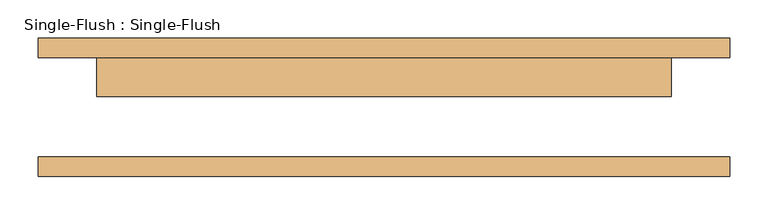
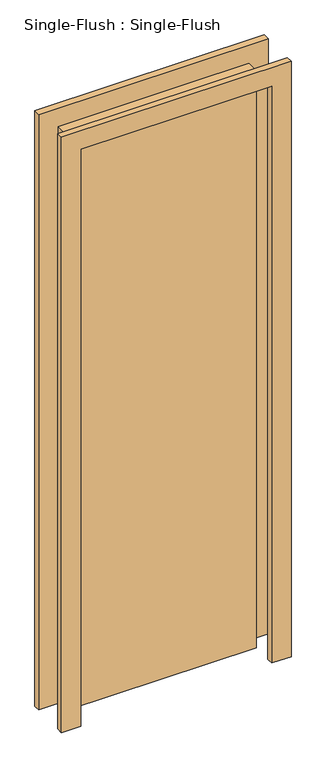
"""IFC4 building model written with IfcOpenShell, lengths in millimetres: door geometry, Single-Flush : Single-Flush."""

import ifcopenshell
import ifcopenshell.guid

model = None  # the IFC model being written
_history = None  # IfcOwnerHistory: only IFC2X3 demands one
_inside = {}  # id of a spatial element -> (the spatial element, [elements in it])
_under = {}  # id of a project, library or spatial element -> (it, [spatial elements below it])
_declared = {}  # id of a project -> (the project, [libraries it declares])
_typed = {}  # id of a type object -> (the type object, [elements of that type])
_made_of = {}  # id of a material, layer set ... -> (it, [elements and type objects made of it])


def new_model(schema):
    """Start an empty IFC model of exactly this schema.

    Asked for "IFC4X3", IfcOpenShell would pick the latest addendum, in which some entities
    have other attributes; the version numbers below select the first issue.
    IFC2X3 requires an IfcOwnerHistory on every rooted entity: one is made here for all.
    """
    global model, _history
    if schema == "IFC4X3":
        model = ifcopenshell.file(schema_version=(4, 3, 0, 0))
    else:
        model = ifcopenshell.file(schema=schema)
    _inside.clear()
    _under.clear()
    _declared.clear()
    _typed.clear()
    _made_of.clear()
    _history = None
    if model.schema == "IFC2X3":
        org = make("IfcOrganization", Name="unknown")
        user = make(
            "IfcPersonAndOrganization",
            ThePerson=make("IfcPerson", FamilyName="unknown"),
            TheOrganization=org,
        )
        app = make(
            "IfcApplication",
            ApplicationDeveloper=org,
            Version="unknown",
            ApplicationFullName="unknown",
            ApplicationIdentifier="unknown",
        )
        _history = make(
            "IfcOwnerHistory",
            OwningUser=user,
            OwningApplication=app,
            ChangeAction="ADDED",
            CreationDate=0,
        )
    return model


def make(cls, **values):
    """One entity of the class cls with the attributes given. An attribute that is None is left unset."""
    return model.create_entity(
        cls, **{name: value for name, value in values.items() if value is not None}
    )


def rooted(cls, **values):
    """An entity with a GlobalId (a new one), such as an element, a storey or a relation."""
    return make(cls, GlobalId=ifcopenshell.guid.new(), OwnerHistory=_history, **values)


def si_unit(unit_type, name, prefix=None):
    """IfcSIUnit, for example si_unit("LENGTHUNIT", "METRE", prefix="MILLI")."""
    return make("IfcSIUnit", UnitType=unit_type, Prefix=prefix, Name=name)


def assignment(units):
    """IfcUnitAssignment: the units of a project."""
    return None if units is None else make("IfcUnitAssignment", Units=units)


def point(xyz):
    """IfcCartesianPoint."""
    return None if xyz is None else make("IfcCartesianPoint", Coordinates=xyz)


def direction(xyz):
    """IfcDirection."""
    return None if xyz is None else make("IfcDirection", DirectionRatios=xyz)


def frame(location, z_axis=None, x_axis=None):
    """IfcAxis2Placement3D, a coordinate frame: its origin and axes. An axis left out is left unset."""
    return make(
        "IfcAxis2Placement3D",
        Location=point(location),
        Axis=direction(z_axis),
        RefDirection=direction(x_axis),
    )


def origin():
    """The frame at (0, 0, 0) with its axes left unset."""
    return frame((0.0, 0.0, 0.0))


def origin_with_axes():
    """The frame at (0, 0, 0) with the z axis (0, 0, 1) and the x axis (1, 0, 0) written out."""
    return frame((0.0, 0.0, 0.0), z_axis=(0.0, 0.0, 1.0), x_axis=(1.0, 0.0, 0.0))


def place(relative_to, where):
    """IfcLocalPlacement: puts the frame where relative to a parent placement (None: the world)."""
    return make(
        "IfcLocalPlacement", PlacementRelTo=relative_to, RelativePlacement=where
    )


def context(
    kind, dimensions, precision=None, world=None, true_north=None, identifier=None
):
    """IfcGeometricRepresentationContext, for example the 3D "Model" context."""
    return make(
        "IfcGeometricRepresentationContext",
        ContextIdentifier=identifier,
        ContextType=kind,
        CoordinateSpaceDimension=dimensions,
        Precision=precision,
        WorldCoordinateSystem=world,
        TrueNorth=true_north,
    )


def project(units=None, contexts=None):
    """IfcProject with its units and contexts."""
    return rooted(
        "IfcProject",
        Name="project",
        RepresentationContexts=contexts,
        UnitsInContext=assignment(units),
    )


def spatial(cls, under=None, at=None, **own):
    """A site, building, storey or space (cls), placed at a placement, below another one or the project."""
    s = rooted(cls, ObjectPlacement=at, **own)
    if under is not None:
        _under.setdefault(under.id(), (under, []))[1].append(s)
    return s


def polyline(points):
    """IfcPolyline through the points."""
    return make("IfcPolyline", Points=[point(p) for p in points])


def outline(outer, holes=None, kind="AREA"):
    """IfcArbitraryClosedProfileDef: a profile drawn as a closed curve; with holes, ...WithVoids."""
    if holes is None:
        return make("IfcArbitraryClosedProfileDef", ProfileType=kind, OuterCurve=outer)
    return make(
        "IfcArbitraryProfileDefWithVoids",
        ProfileType=kind,
        OuterCurve=outer,
        InnerCurves=holes,
    )


def extrude(swept, where, along, depth):
    """IfcExtrudedAreaSolid: the profile swept, set in the frame where, extruded along a direction by depth."""
    return make(
        "IfcExtrudedAreaSolid",
        SweptArea=swept,
        Position=where,
        ExtrudedDirection=direction(along),
        Depth=depth,
    )


def shape(context_of_items, identifier, shape_type, items):
    """IfcShapeRepresentation: the items that make up one representation, for example the "Body"."""
    return make(
        "IfcShapeRepresentation",
        ContextOfItems=context_of_items,
        RepresentationIdentifier=identifier,
        RepresentationType=shape_type,
        Items=items,
    )


def source(mapping_origin, context_of_items, identifier, shape_type, items):
    """IfcRepresentationMap: a shape defined once, which mapped items show again and again."""
    return make(
        "IfcRepresentationMap",
        MappingOrigin=mapping_origin,
        MappedRepresentation=shape(context_of_items, identifier, shape_type, items),
    )


def transform(
    local_origin,
    x_axis=None,
    y_axis=None,
    z_axis=None,
    scale=None,
    scale2=None,
    scale3=None,
    uniform=True,
):
    """IfcCartesianTransformationOperator3D, or its non-uniform kind. x_axis, y_axis, z_axis: its Axis1, 2, 3."""
    if uniform:
        return make(
            "IfcCartesianTransformationOperator3D",
            Axis1=direction(x_axis),
            Axis2=direction(y_axis),
            LocalOrigin=point(local_origin),
            Scale=scale,
            Axis3=direction(z_axis),
        )
    return make(
        "IfcCartesianTransformationOperator3DnonUniform",
        Axis1=direction(x_axis),
        Axis2=direction(y_axis),
        LocalOrigin=point(local_origin),
        Scale=scale,
        Axis3=direction(z_axis),
        Scale2=scale2,
        Scale3=scale3,
    )


def mapped(mapping_source, mapping_target):
    """IfcMappedItem: shows the shape of a source again, moved by a transform."""
    return make(
        "IfcMappedItem", MappingSource=mapping_source, MappingTarget=mapping_target
    )


def made_of(thing, what):
    """Note that an element or type object is made of a material, layer set ...; save() writes the relation."""
    if what is not None:
        _made_of.setdefault(what.id(), (what, []))[1].append(thing)
    return thing


def element(
    cls,
    number,
    at=None,
    inside=None,
    cuts=None,
    type_object=None,
    material=None,
    context=None,
    identifier="Body",
    shape_type=None,
    held_by="IfcProductDefinitionShape",
    body=None,
    shapes=None,
    **own,
):
    """One element of the class cls, such as IfcWall. Its Tag is "e" and its number.

    at: its placement. inside: the storey or other place that contains it. cuts: it is an
    opening in that element (IfcRelVoidsElement). A single representation is given by context,
    identifier, shape_type and body (its items); several are given by shapes. held_by: the class
    of the entity that holds the representations. save() writes the other relations.
    """
    e = rooted(cls, Tag="e%d" % number, ObjectPlacement=at, **own)
    if body is not None:
        shapes = [shape(context, identifier, shape_type, body)]
    if shapes is not None:
        e.Representation = make(held_by, Representations=shapes)
    if inside is not None:
        _inside.setdefault(inside.id(), (inside, []))[1].append(e)
    if cuts is not None:
        rooted(
            "IfcRelVoidsElement", RelatingBuildingElement=cuts, RelatedOpeningElement=e
        )
    if type_object is not None:
        _typed.setdefault(type_object.id(), (type_object, []))[1].append(e)
    return made_of(e, material)


def aggregate(whole, parts):
    """IfcRelAggregates: a whole, such as a stair, and the parts it consists of."""
    return rooted("IfcRelAggregates", RelatingObject=whole, RelatedObjects=parts)


def save(model, path):
    """Write the relations noted so far, then the file.

    IfcRelAggregates (storeys below a building ...), IfcRelContainedInSpatialStructure (elements
    in a storey), IfcRelDefinesByType, IfcRelAssociatesMaterial and IfcRelDeclares: one each for
    every whole, place, type object, material and project.
    """
    for whole, parts in _under.values():
        aggregate(whole, parts)
    for where, things in _inside.values():
        rooted(
            "IfcRelContainedInSpatialStructure",
            RelatedElements=things,
            RelatingStructure=where,
        )
    for kind, things in _typed.values():
        rooted("IfcRelDefinesByType", RelatedObjects=things, RelatingType=kind)
    for what, things in _made_of.values():
        rooted("IfcRelAssociatesMaterial", RelatedObjects=things, RelatingMaterial=what)
    for by, libraries in _declared.values():
        rooted("IfcRelDeclares", RelatingContext=by, RelatedDefinitions=libraries)
    model.write(path)


def single_flush_single_flush_4c6b4bcb(model_context):
    return source(origin(), model_context, "Body", "SweptSolid", [
        extrude(outline(polyline([(375.0, 14.2), (-375.0, 14.2), (-375.0, 65.0), (375.0, 65.0), (375.0, 14.2)])), origin_with_axes(), (0.0, 0.0, 1.0), 2400.0),
        extrude(outline(polyline([(2476.2, 451.2), (2476.2, -451.2), (0.0, -451.2), (0.0, -375.0), (2400.0, -375.0), (2400.0, 375.0), (0.0, 375.0), (0.0, 451.2), (2476.2, 451.2)])), frame((0.0, -90.4, 0.0), z_axis=(0.0, 1.0, 0.0), x_axis=(0.0, 0.0, 1.0)), (0.0, 0.0, 1.0), 25.4),
        extrude(outline(polyline([(2476.2, -451.2), (0.0, -451.2), (0.0, -375.0), (2400.0, -375.0), (2400.0, 375.0), (0.0, 375.0), (0.0, 451.2), (2476.2, 451.2), (2476.2, -451.2)])), frame((0.0, 65.0, 0.0), z_axis=(0.0, 1.0, 0.0), x_axis=(0.0, 0.0, 1.0)), (0.0, 0.0, 1.0), 25.4),
    ])


if __name__ == "__main__":
    model = new_model("IFC4")
    model_context = context("Model", 3, world=origin())
    ifc_project = project(units=[si_unit("LENGTHUNIT", "METRE", prefix="MILLI")], contexts=[model_context])
    site = spatial("IfcSite", under=ifc_project)
    building = spatial("IfcBuilding", under=site)
    placement = place(None, origin())
    single_flush_single_flush_shape = single_flush_single_flush_4c6b4bcb(model_context)
    element("IfcDoor", 1, ObjectType="Single-Flush : Single-Flush", at=placement, inside=building, context=model_context, shape_type="MappedRepresentation", body=[
        mapped(single_flush_single_flush_shape, transform((0.0, 0.0, 0.0), x_axis=(1.0, 0.0, 0.0), y_axis=(0.0, 1.0, 0.0), z_axis=(0.0, 0.0, 1.0))),
    ])
    save(model, "model.ifc")

# Revit data of these elements
# Type "Single-Flush : Single-Flush"
#   Type Mark = "61"
#   Assembly Code = "C1020"
#   Analytic Construction = "<None>"
#   Thickness = 50.8 mm
#   Height = 2400 mm
#   Trim Projection Ext = 25.4 mm
#   Trim Projection Int = 25.4 mm
#   Trim Width = 76.2 mm
#   Width = 750 mm
#   Define Thermal Properties by = 1
#   Door Material = Door - Panel
#   Frame Material = Door - Frame
#   Function = (empty or 0)
#   Wall Closure = (empty or 0)
# Element 1 (IfcDoor, "Single-Flush : Single-Flush")
#   Materials on its faces: "Door - Frame", "Door - Panel"
# Materials
#   "Door - Panel": class "Wood", colour RGB 210 159 95, transparency 0, Cost = 0
#   "Door - Frame": class "Unassigned", colour RGB 118 70 51, transparency 0, Keynote = "L20"
